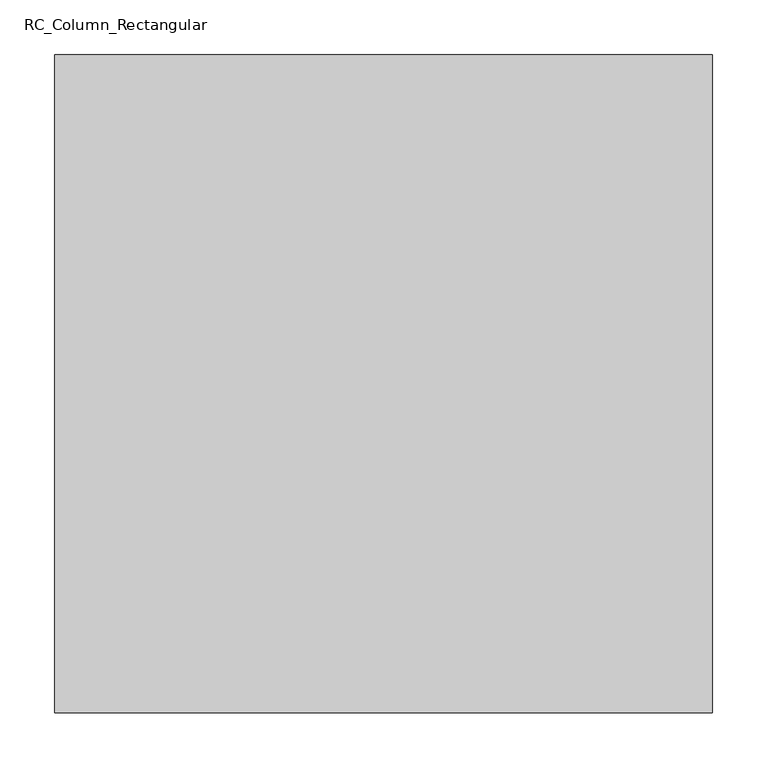
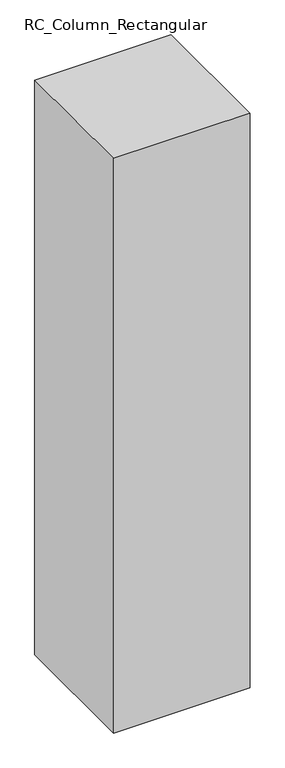
"""IFC4 building model written with IfcOpenShell, lengths in millimetres: column geometry, RC_Column_Rectangular : H_SC_AR_S15_W600xL600."""

import ifcopenshell
import ifcopenshell.guid

model = None  # the IFC model being written
_history = None  # IfcOwnerHistory: only IFC2X3 demands one
_inside = {}  # id of a spatial element -> (the spatial element, [elements in it])
_under = {}  # id of a project, library or spatial element -> (it, [spatial elements below it])
_declared = {}  # id of a project -> (the project, [libraries it declares])
_typed = {}  # id of a type object -> (the type object, [elements of that type])
_made_of = {}  # id of a material, layer set ... -> (it, [elements and type objects made of it])


def new_model(schema):
    """Start an empty IFC model of exactly this schema.

    Asked for "IFC4X3", IfcOpenShell would pick the latest addendum, in which some entities
    have other attributes; the version numbers below select the first issue.
    IFC2X3 requires an IfcOwnerHistory on every rooted entity: one is made here for all.
    """
    global model, _history
    if schema == "IFC4X3":
        model = ifcopenshell.file(schema_version=(4, 3, 0, 0))
    else:
        model = ifcopenshell.file(schema=schema)
    _inside.clear()
    _under.clear()
    _declared.clear()
    _typed.clear()
    _made_of.clear()
    _history = None
    if model.schema == "IFC2X3":
        org = make("IfcOrganization", Name="unknown")
        user = make(
            "IfcPersonAndOrganization",
            ThePerson=make("IfcPerson", FamilyName="unknown"),
            TheOrganization=org,
        )
        app = make(
            "IfcApplication",
            ApplicationDeveloper=org,
            Version="unknown",
            ApplicationFullName="unknown",
            ApplicationIdentifier="unknown",
        )
        _history = make(
            "IfcOwnerHistory",
            OwningUser=user,
            OwningApplication=app,
            ChangeAction="ADDED",
            CreationDate=0,
        )
    return model


def make(cls, **values):
    """One entity of the class cls with the attributes given. An attribute that is None is left unset."""
    return model.create_entity(
        cls, **{name: value for name, value in values.items() if value is not None}
    )


def rooted(cls, **values):
    """An entity with a GlobalId (a new one), such as an element, a storey or a relation."""
    return make(cls, GlobalId=ifcopenshell.guid.new(), OwnerHistory=_history, **values)


def si_unit(unit_type, name, prefix=None):
    """IfcSIUnit, for example si_unit("LENGTHUNIT", "METRE", prefix="MILLI")."""
    return make("IfcSIUnit", UnitType=unit_type, Prefix=prefix, Name=name)


def assignment(units):
    """IfcUnitAssignment: the units of a project."""
    return None if units is None else make("IfcUnitAssignment", Units=units)


def point(xyz):
    """IfcCartesianPoint."""
    return None if xyz is None else make("IfcCartesianPoint", Coordinates=xyz)


def direction(xyz):
    """IfcDirection."""
    return None if xyz is None else make("IfcDirection", DirectionRatios=xyz)


def frame(location, z_axis=None, x_axis=None):
    """IfcAxis2Placement3D, a coordinate frame: its origin and axes. An axis left out is left unset."""
    return make(
        "IfcAxis2Placement3D",
        Location=point(location),
        Axis=direction(z_axis),
        RefDirection=direction(x_axis),
    )


def origin():
    """The frame at (0, 0, 0) with its axes left unset."""
    return frame((0.0, 0.0, 0.0))


def place(relative_to, where):
    """IfcLocalPlacement: puts the frame where relative to a parent placement (None: the world)."""
    return make(
        "IfcLocalPlacement", PlacementRelTo=relative_to, RelativePlacement=where
    )


def context(
    kind, dimensions, precision=None, world=None, true_north=None, identifier=None
):
    """IfcGeometricRepresentationContext, for example the 3D "Model" context."""
    return make(
        "IfcGeometricRepresentationContext",
        ContextIdentifier=identifier,
        ContextType=kind,
        CoordinateSpaceDimension=dimensions,
        Precision=precision,
        WorldCoordinateSystem=world,
        TrueNorth=true_north,
    )


def project(units=None, contexts=None):
    """IfcProject with its units and contexts."""
    return rooted(
        "IfcProject",
        Name="project",
        RepresentationContexts=contexts,
        UnitsInContext=assignment(units),
    )


def spatial(cls, under=None, at=None, **own):
    """A site, building, storey or space (cls), placed at a placement, below another one or the project."""
    s = rooted(cls, ObjectPlacement=at, **own)
    if under is not None:
        _under.setdefault(under.id(), (under, []))[1].append(s)
    return s


def polyline(points):
    """IfcPolyline through the points."""
    return make("IfcPolyline", Points=[point(p) for p in points])


def outline(outer, holes=None, kind="AREA"):
    """IfcArbitraryClosedProfileDef: a profile drawn as a closed curve; with holes, ...WithVoids."""
    if holes is None:
        return make("IfcArbitraryClosedProfileDef", ProfileType=kind, OuterCurve=outer)
    return make(
        "IfcArbitraryProfileDefWithVoids",
        ProfileType=kind,
        OuterCurve=outer,
        InnerCurves=holes,
    )


def extrude(swept, where, along, depth):
    """IfcExtrudedAreaSolid: the profile swept, set in the frame where, extruded along a direction by depth."""
    return make(
        "IfcExtrudedAreaSolid",
        SweptArea=swept,
        Position=where,
        ExtrudedDirection=direction(along),
        Depth=depth,
    )


def shape(context_of_items, identifier, shape_type, items):
    """IfcShapeRepresentation: the items that make up one representation, for example the "Body"."""
    return make(
        "IfcShapeRepresentation",
        ContextOfItems=context_of_items,
        RepresentationIdentifier=identifier,
        RepresentationType=shape_type,
        Items=items,
    )


def source(mapping_origin, context_of_items, identifier, shape_type, items):
    """IfcRepresentationMap: a shape defined once, which mapped items show again and again."""
    return make(
        "IfcRepresentationMap",
        MappingOrigin=mapping_origin,
        MappedRepresentation=shape(context_of_items, identifier, shape_type, items),
    )


def transform(
    local_origin,
    x_axis=None,
    y_axis=None,
    z_axis=None,
    scale=None,
    scale2=None,
    scale3=None,
    uniform=True,
):
    """IfcCartesianTransformationOperator3D, or its non-uniform kind. x_axis, y_axis, z_axis: its Axis1, 2, 3."""
    if uniform:
        return make(
            "IfcCartesianTransformationOperator3D",
            Axis1=direction(x_axis),
            Axis2=direction(y_axis),
            LocalOrigin=point(local_origin),
            Scale=scale,
            Axis3=direction(z_axis),
        )
    return make(
        "IfcCartesianTransformationOperator3DnonUniform",
        Axis1=direction(x_axis),
        Axis2=direction(y_axis),
        LocalOrigin=point(local_origin),
        Scale=scale,
        Axis3=direction(z_axis),
        Scale2=scale2,
        Scale3=scale3,
    )


def mapped(mapping_source, mapping_target):
    """IfcMappedItem: shows the shape of a source again, moved by a transform."""
    return make(
        "IfcMappedItem", MappingSource=mapping_source, MappingTarget=mapping_target
    )


def made_of(thing, what):
    """Note that an element or type object is made of a material, layer set ...; save() writes the relation."""
    if what is not None:
        _made_of.setdefault(what.id(), (what, []))[1].append(thing)
    return thing


def element(
    cls,
    number,
    at=None,
    inside=None,
    cuts=None,
    type_object=None,
    material=None,
    context=None,
    identifier="Body",
    shape_type=None,
    held_by="IfcProductDefinitionShape",
    body=None,
    shapes=None,
    **own,
):
    """One element of the class cls, such as IfcWall. Its Tag is "e" and its number.

    at: its placement. inside: the storey or other place that contains it. cuts: it is an
    opening in that element (IfcRelVoidsElement). A single representation is given by context,
    identifier, shape_type and body (its items); several are given by shapes. held_by: the class
    of the entity that holds the representations. save() writes the other relations.
    """
    e = rooted(cls, Tag="e%d" % number, ObjectPlacement=at, **own)
    if body is not None:
        shapes = [shape(context, identifier, shape_type, body)]
    if shapes is not None:
        e.Representation = make(held_by, Representations=shapes)
    if inside is not None:
        _inside.setdefault(inside.id(), (inside, []))[1].append(e)
    if cuts is not None:
        rooted(
            "IfcRelVoidsElement", RelatingBuildingElement=cuts, RelatedOpeningElement=e
        )
    if type_object is not None:
        _typed.setdefault(type_object.id(), (type_object, []))[1].append(e)
    return made_of(e, material)


def aggregate(whole, parts):
    """IfcRelAggregates: a whole, such as a stair, and the parts it consists of."""
    return rooted("IfcRelAggregates", RelatingObject=whole, RelatedObjects=parts)


def save(model, path):
    """Write the relations noted so far, then the file.

    IfcRelAggregates (storeys below a building ...), IfcRelContainedInSpatialStructure (elements
    in a storey), IfcRelDefinesByType, IfcRelAssociatesMaterial and IfcRelDeclares: one each for
    every whole, place, type object, material and project.
    """
    for whole, parts in _under.values():
        aggregate(whole, parts)
    for where, things in _inside.values():
        rooted(
            "IfcRelContainedInSpatialStructure",
            RelatedElements=things,
            RelatingStructure=where,
        )
    for kind, things in _typed.values():
        rooted("IfcRelDefinesByType", RelatedObjects=things, RelatingType=kind)
    for what, things in _made_of.values():
        rooted("IfcRelAssociatesMaterial", RelatedObjects=things, RelatingMaterial=what)
    for by, libraries in _declared.values():
        rooted("IfcRelDeclares", RelatingContext=by, RelatedDefinitions=libraries)
    model.write(path)


def rc_column_rectangular_090fd146(model_context):
    return source(origin(), model_context, "Body", "SweptSolid", [
        extrude(outline(polyline([(300.0, 300.0), (300.0, -300.0), (-300.0, -300.0), (-300.0, 300.0), (300.0, 300.0)])), frame((0.0, 0.0, 11309.9618634), z_axis=(0.0, 0.0, 1.0), x_axis=(1.0, 0.0, 0.0)), (0.0, 0.0, 1.0), 2670.0),
    ])


if __name__ == "__main__":
    model = new_model("IFC4")
    model_context = context("Model", 3, world=origin())
    ifc_project = project(units=[si_unit("LENGTHUNIT", "METRE", prefix="MILLI")], contexts=[model_context])
    site = spatial("IfcSite", under=ifc_project)
    building = spatial("IfcBuilding", under=site)
    placement = place(None, origin())
    rc_column_rectangular_shape = rc_column_rectangular_090fd146(model_context)
    element("IfcColumn", 1, ObjectType="RC_Column_Rectangular : H_SC_AR_S15_W600xL600", at=placement, inside=building, context=model_context, shape_type="MappedRepresentation", body=[
        mapped(rc_column_rectangular_shape, transform((0.0, 0.0, 0.0), x_axis=(1.0, 0.0, 0.0), y_axis=(0.0, 1.0, 0.0), z_axis=(0.0, 0.0, 1.0))),
    ])
    save(model, "model.ifc")

# Revit data of these elements
# Type "RC_Column_Rectangular : H_SC_AR_S15_W600xL600"
#   Width = 600 mm
#   Length = 600 mm
#   hec_material3 [instance default] = none
#   hec_material2 [instance default] = none
#   hec_material1 [instance default] = none
#   Structural Material [instance default] = none
#   Description = (empty or 0)
